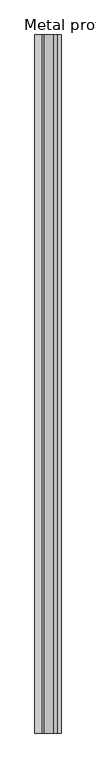
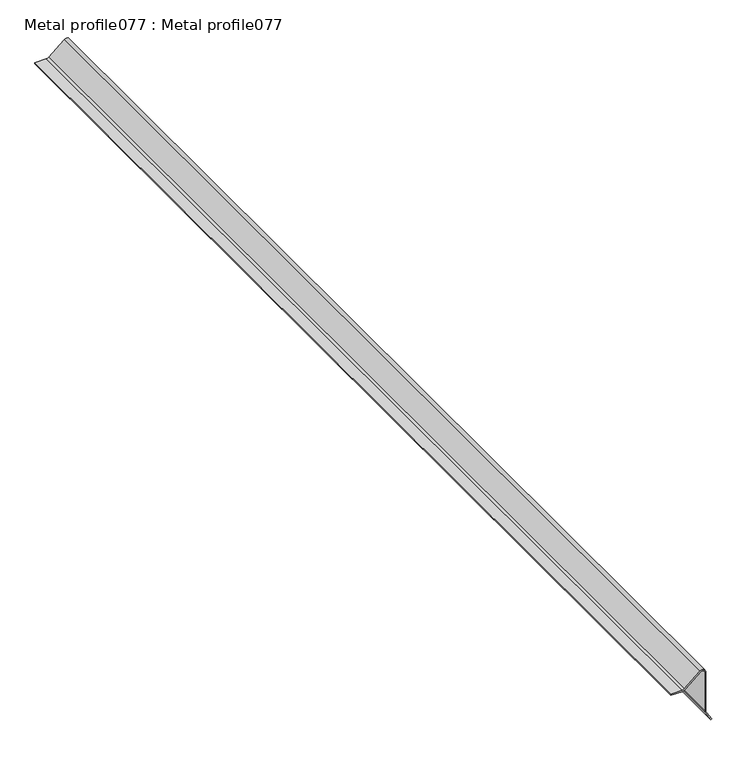
"""IFC4 building model written with IfcOpenShell, lengths in millimetres: proxy geometry, Metal profile077 : Metal profile077."""

from ifc_helpers import new_model, si_unit, point, frame, frame_2d, origin, place, context, project, spatial, polyline, circle_curve, trimmed, segment, composite_curve, outline, extrude, source, transform, mapped, element, save


def metal_profile077_metal_profile077_44bae506(model_context):
    return source(origin(), model_context, "Body", "SweptSolid", [
        extrude(outline(composite_curve([segment(polyline([(40167.3242187, -9308.0342101), (40167.3242187, -9329.0017486), (40165.3242188, -9329.0017486), (40165.3242187, -9308.0342101)]), True, "CONTINUOUS"), segment(trimmed(circle_curve(frame_2d((40173.6742187, -9308.0342101)), 8.35), [point((40165.3242187, -9308.0342101))], [point((40167.3459716, -9302.5866613))], False, "CARTESIAN"), True, "CONTINUOUS"), segment(polyline([(40167.3459716, -9302.5866613), (40191.4908371, -9274.538326)]), True, "CONTINUOUS"), segment(trimmed(circle_curve(frame_2d((40188.1940856, -9271.7003814)), 4.35), [point((40191.4908371, -9274.538326))], [point((40188.1940856, -9267.3503814))], True, "CARTESIAN"), True, "CONTINUOUS"), segment(polyline([(40188.1940856, -9267.3503814), (40113.9784377, -9267.3503814)]), True, "CONTINUOUS"), segment(trimmed(circle_curve(frame_2d((40113.9784377, -9259.0003814)), 8.35), [point((40113.9784377, -9267.3503814))], [point((40109.5830768, -9266.0999098))], False, "CARTESIAN"), True, "CONTINUOUS"), segment(polyline([(40109.5830768, -9266.0999098), (40092.8105002, -9255.7159063), (40093.8632812, -9254.0154205), (40110.6358579, -9264.3994239)]), True, "CONTINUOUS"), segment(trimmed(circle_curve(frame_2d((40113.9784377, -9259.0003814)), 6.35), [point((40110.6358579, -9264.3994239))], [point((40113.9784377, -9265.3503814))], True, "CARTESIAN"), True, "CONTINUOUS"), segment(polyline([(40113.9784377, -9265.3503814), (40188.1940856, -9265.3503814)]), True, "CONTINUOUS"), segment(trimmed(circle_curve(frame_2d((40188.1940856, -9271.7003814)), 6.35), [point((40188.1940856, -9265.3503814))], [point((40193.006585, -9275.8431281))], False, "CARTESIAN"), True, "CONTINUOUS"), segment(polyline([(40193.006585, -9275.8431281), (40168.8617194, -9303.8914634)]), True, "CONTINUOUS"), segment(trimmed(circle_curve(frame_2d((40173.6742187, -9308.0342101)), 6.35), [point((40168.8617194, -9303.8914634))], [point((40167.3242187, -9308.0342101))], True, "CARTESIAN"), True, "CONTINUOUS")], self_intersect=False)), frame((0.0, 7982.1531721, 0.0), z_axis=(0.0, 1.0, 0.0), x_axis=(0.0, 0.0, 1.0)), (0.0, 0.0, 1.0), 2000.0),
    ])


if __name__ == "__main__":
    model = new_model("IFC4")
    model_context = context("Model", 3, world=origin())
    ifc_project = project(units=[si_unit("LENGTHUNIT", "METRE", prefix="MILLI")], contexts=[model_context])
    site = spatial("IfcSite", under=ifc_project)
    building = spatial("IfcBuilding", under=site)
    placement = place(None, origin())
    metal_profile077_metal_profile077_shape = metal_profile077_metal_profile077_44bae506(model_context)
    element("IfcBuildingElementProxy", 1, Name="Metal profile077 : Metal profile077", ObjectType="Metal profile077 : Metal profile077", at=placement, inside=building, context=model_context, shape_type="MappedRepresentation", body=[
        mapped(metal_profile077_metal_profile077_shape, transform((0.0, 0.0, 0.0), x_axis=(1.0, 0.0, 0.0), y_axis=(0.0, 1.0, 0.0), z_axis=(0.0, 0.0, 1.0))),
    ])
    save(model, "model.ifc")

# Revit data of these elements
# Type "Metal profile077 : Metal profile077"
#   NameOverride = "Metal profile077"
# Element 1 (IfcBuildingElementProxy, "Metal profile077 : Metal profile077")
#   Materials on its faces: "ANGLE TRIM"
# Materials
#   "ANGLE TRIM": class "Unassigned", colour RGB 250 255 0, transparency 0
